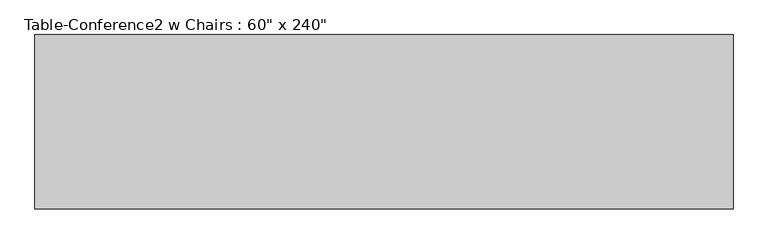
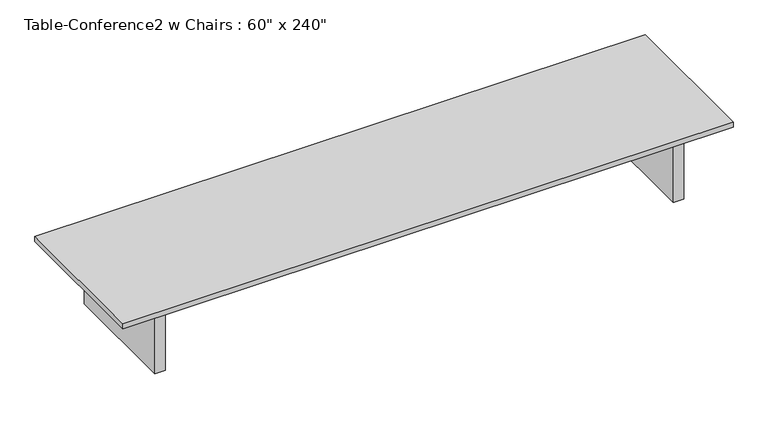
"""IFC4 building model written with IfcOpenShell, lengths in millimetres: furniture geometry."""

import ifcopenshell
import ifcopenshell.guid

model = None  # the IFC model being written
_history = None  # IfcOwnerHistory: only IFC2X3 demands one
_inside = {}  # id of a spatial element -> (the spatial element, [elements in it])
_under = {}  # id of a project, library or spatial element -> (it, [spatial elements below it])
_declared = {}  # id of a project -> (the project, [libraries it declares])
_typed = {}  # id of a type object -> (the type object, [elements of that type])
_made_of = {}  # id of a material, layer set ... -> (it, [elements and type objects made of it])


def new_model(schema):
    """Start an empty IFC model of exactly this schema.

    Asked for "IFC4X3", IfcOpenShell would pick the latest addendum, in which some entities
    have other attributes; the version numbers below select the first issue.
    IFC2X3 requires an IfcOwnerHistory on every rooted entity: one is made here for all.
    """
    global model, _history
    if schema == "IFC4X3":
        model = ifcopenshell.file(schema_version=(4, 3, 0, 0))
    else:
        model = ifcopenshell.file(schema=schema)
    _inside.clear()
    _under.clear()
    _declared.clear()
    _typed.clear()
    _made_of.clear()
    _history = None
    if model.schema == "IFC2X3":
        org = make("IfcOrganization", Name="unknown")
        user = make(
            "IfcPersonAndOrganization",
            ThePerson=make("IfcPerson", FamilyName="unknown"),
            TheOrganization=org,
        )
        app = make(
            "IfcApplication",
            ApplicationDeveloper=org,
            Version="unknown",
            ApplicationFullName="unknown",
            ApplicationIdentifier="unknown",
        )
        _history = make(
            "IfcOwnerHistory",
            OwningUser=user,
            OwningApplication=app,
            ChangeAction="ADDED",
            CreationDate=0,
        )
    return model


def make(cls, **values):
    """One entity of the class cls with the attributes given. An attribute that is None is left unset."""
    return model.create_entity(
        cls, **{name: value for name, value in values.items() if value is not None}
    )


def rooted(cls, **values):
    """An entity with a GlobalId (a new one), such as an element, a storey or a relation."""
    return make(cls, GlobalId=ifcopenshell.guid.new(), OwnerHistory=_history, **values)


def si_unit(unit_type, name, prefix=None):
    """IfcSIUnit, for example si_unit("LENGTHUNIT", "METRE", prefix="MILLI")."""
    return make("IfcSIUnit", UnitType=unit_type, Prefix=prefix, Name=name)


def assignment(units):
    """IfcUnitAssignment: the units of a project."""
    return None if units is None else make("IfcUnitAssignment", Units=units)


def point(xyz):
    """IfcCartesianPoint."""
    return None if xyz is None else make("IfcCartesianPoint", Coordinates=xyz)


def direction(xyz):
    """IfcDirection."""
    return None if xyz is None else make("IfcDirection", DirectionRatios=xyz)


def frame(location, z_axis=None, x_axis=None):
    """IfcAxis2Placement3D, a coordinate frame: its origin and axes. An axis left out is left unset."""
    return make(
        "IfcAxis2Placement3D",
        Location=point(location),
        Axis=direction(z_axis),
        RefDirection=direction(x_axis),
    )


def origin():
    """The frame at (0, 0, 0) with its axes left unset."""
    return frame((0.0, 0.0, 0.0))


def origin_with_axes():
    """The frame at (0, 0, 0) with the z axis (0, 0, 1) and the x axis (1, 0, 0) written out."""
    return frame((0.0, 0.0, 0.0), z_axis=(0.0, 0.0, 1.0), x_axis=(1.0, 0.0, 0.0))


def place(relative_to, where):
    """IfcLocalPlacement: puts the frame where relative to a parent placement (None: the world)."""
    return make(
        "IfcLocalPlacement", PlacementRelTo=relative_to, RelativePlacement=where
    )


def context(
    kind, dimensions, precision=None, world=None, true_north=None, identifier=None
):
    """IfcGeometricRepresentationContext, for example the 3D "Model" context."""
    return make(
        "IfcGeometricRepresentationContext",
        ContextIdentifier=identifier,
        ContextType=kind,
        CoordinateSpaceDimension=dimensions,
        Precision=precision,
        WorldCoordinateSystem=world,
        TrueNorth=true_north,
    )


def project(units=None, contexts=None):
    """IfcProject with its units and contexts."""
    return rooted(
        "IfcProject",
        Name="project",
        RepresentationContexts=contexts,
        UnitsInContext=assignment(units),
    )


def spatial(cls, under=None, at=None, **own):
    """A site, building, storey or space (cls), placed at a placement, below another one or the project."""
    s = rooted(cls, ObjectPlacement=at, **own)
    if under is not None:
        _under.setdefault(under.id(), (under, []))[1].append(s)
    return s


def polyline(points):
    """IfcPolyline through the points."""
    return make("IfcPolyline", Points=[point(p) for p in points])


def outline(outer, holes=None, kind="AREA"):
    """IfcArbitraryClosedProfileDef: a profile drawn as a closed curve; with holes, ...WithVoids."""
    if holes is None:
        return make("IfcArbitraryClosedProfileDef", ProfileType=kind, OuterCurve=outer)
    return make(
        "IfcArbitraryProfileDefWithVoids",
        ProfileType=kind,
        OuterCurve=outer,
        InnerCurves=holes,
    )


def extrude(swept, where, along, depth):
    """IfcExtrudedAreaSolid: the profile swept, set in the frame where, extruded along a direction by depth."""
    return make(
        "IfcExtrudedAreaSolid",
        SweptArea=swept,
        Position=where,
        ExtrudedDirection=direction(along),
        Depth=depth,
    )


def shape(context_of_items, identifier, shape_type, items):
    """IfcShapeRepresentation: the items that make up one representation, for example the "Body"."""
    return make(
        "IfcShapeRepresentation",
        ContextOfItems=context_of_items,
        RepresentationIdentifier=identifier,
        RepresentationType=shape_type,
        Items=items,
    )


def source(mapping_origin, context_of_items, identifier, shape_type, items):
    """IfcRepresentationMap: a shape defined once, which mapped items show again and again."""
    return make(
        "IfcRepresentationMap",
        MappingOrigin=mapping_origin,
        MappedRepresentation=shape(context_of_items, identifier, shape_type, items),
    )


def transform(
    local_origin,
    x_axis=None,
    y_axis=None,
    z_axis=None,
    scale=None,
    scale2=None,
    scale3=None,
    uniform=True,
):
    """IfcCartesianTransformationOperator3D, or its non-uniform kind. x_axis, y_axis, z_axis: its Axis1, 2, 3."""
    if uniform:
        return make(
            "IfcCartesianTransformationOperator3D",
            Axis1=direction(x_axis),
            Axis2=direction(y_axis),
            LocalOrigin=point(local_origin),
            Scale=scale,
            Axis3=direction(z_axis),
        )
    return make(
        "IfcCartesianTransformationOperator3DnonUniform",
        Axis1=direction(x_axis),
        Axis2=direction(y_axis),
        LocalOrigin=point(local_origin),
        Scale=scale,
        Axis3=direction(z_axis),
        Scale2=scale2,
        Scale3=scale3,
    )


def mapped(mapping_source, mapping_target):
    """IfcMappedItem: shows the shape of a source again, moved by a transform."""
    return make(
        "IfcMappedItem", MappingSource=mapping_source, MappingTarget=mapping_target
    )


def made_of(thing, what):
    """Note that an element or type object is made of a material, layer set ...; save() writes the relation."""
    if what is not None:
        _made_of.setdefault(what.id(), (what, []))[1].append(thing)
    return thing


def element(
    cls,
    number,
    at=None,
    inside=None,
    cuts=None,
    type_object=None,
    material=None,
    context=None,
    identifier="Body",
    shape_type=None,
    held_by="IfcProductDefinitionShape",
    body=None,
    shapes=None,
    **own,
):
    """One element of the class cls, such as IfcWall. Its Tag is "e" and its number.

    at: its placement. inside: the storey or other place that contains it. cuts: it is an
    opening in that element (IfcRelVoidsElement). A single representation is given by context,
    identifier, shape_type and body (its items); several are given by shapes. held_by: the class
    of the entity that holds the representations. save() writes the other relations.
    """
    e = rooted(cls, Tag="e%d" % number, ObjectPlacement=at, **own)
    if body is not None:
        shapes = [shape(context, identifier, shape_type, body)]
    if shapes is not None:
        e.Representation = make(held_by, Representations=shapes)
    if inside is not None:
        _inside.setdefault(inside.id(), (inside, []))[1].append(e)
    if cuts is not None:
        rooted(
            "IfcRelVoidsElement", RelatingBuildingElement=cuts, RelatedOpeningElement=e
        )
    if type_object is not None:
        _typed.setdefault(type_object.id(), (type_object, []))[1].append(e)
    return made_of(e, material)


def aggregate(whole, parts):
    """IfcRelAggregates: a whole, such as a stair, and the parts it consists of."""
    return rooted("IfcRelAggregates", RelatingObject=whole, RelatedObjects=parts)


def save(model, path):
    """Write the relations noted so far, then the file.

    IfcRelAggregates (storeys below a building ...), IfcRelContainedInSpatialStructure (elements
    in a storey), IfcRelDefinesByType, IfcRelAssociatesMaterial and IfcRelDeclares: one each for
    every whole, place, type object, material and project.
    """
    for whole, parts in _under.values():
        aggregate(whole, parts)
    for where, things in _inside.values():
        rooted(
            "IfcRelContainedInSpatialStructure",
            RelatedElements=things,
            RelatingStructure=where,
        )
    for kind, things in _typed.values():
        rooted("IfcRelDefinesByType", RelatedObjects=things, RelatingType=kind)
    for what, things in _made_of.values():
        rooted("IfcRelAssociatesMaterial", RelatedObjects=things, RelatingMaterial=what)
    for by, libraries in _declared.values():
        rooted("IfcRelDeclares", RelatingContext=by, RelatedDefinitions=libraries)
    model.write(path)


def furniture_b1813a45(model_context):
    return source(origin(), model_context, "Body", "SweptSolid", [
        extrude(outline(polyline([(2540.0, 609.6), (2540.0, 571.5), (-2540.0, 571.5), (-2540.0, 609.6), (2540.0, 609.6)])), frame((0.0, 0.0, 609.6), z_axis=(0.0, 0.0, 1.0), x_axis=(1.0, 0.0, 0.0)), (0.0, 0.0, 1.0), 101.6),
        extrude(outline(polyline([(2540.0, -609.6), (-2540.0, -609.6), (-2540.0, -571.5), (2540.0, -571.5), (2540.0, -609.6)])), frame((0.0, 0.0, 609.6), z_axis=(0.0, 0.0, 1.0), x_axis=(1.0, 0.0, 0.0)), (0.0, 0.0, 1.0), 101.6),
        extrude(outline(polyline([(-2540.0, -609.6), (-2641.6, -609.6), (-2641.6, 609.6), (-2540.0, 609.6), (-2540.0, -609.6)])), origin_with_axes(), (0.0, 0.0, 1.0), 711.2),
        extrude(outline(polyline([(2641.6, -609.6), (2540.0, -609.6), (2540.0, 609.6), (2641.6, 609.6), (2641.6, -609.6)])), origin_with_axes(), (0.0, 0.0, 1.0), 711.2),
        extrude(outline(polyline([(3048.0, -762.0), (-3048.0, -762.0), (-3048.0, 762.0), (3048.0, 762.0), (3048.0, -762.0)])), frame((0.0, 0.0, 711.2), z_axis=(0.0, 0.0, 1.0), x_axis=(1.0, 0.0, 0.0)), (0.0, 0.0, 1.0), 50.8),
    ])


if __name__ == "__main__":
    model = new_model("IFC4")
    model_context = context("Model", 3, world=origin())
    ifc_project = project(units=[si_unit("LENGTHUNIT", "METRE", prefix="MILLI")], contexts=[model_context])
    site = spatial("IfcSite", under=ifc_project)
    building = spatial("IfcBuilding", under=site)
    placement = place(None, origin())
    furniture_shape = furniture_b1813a45(model_context)
    element("IfcFurniture", 1, ObjectType="Table-Conference2 w Chairs : 60\" x 240\"", at=placement, inside=building, context=model_context, shape_type="MappedRepresentation", body=[
        mapped(furniture_shape, transform((0.0, 0.0, 0.0), x_axis=(1.0, 0.0, 0.0), y_axis=(0.0, 1.0, 0.0), z_axis=(0.0, 0.0, 1.0))),
    ])
    save(model, "model.ifc")

# Revit data of these elements
# Type "Table-Conference2 w Chairs : 60\" x 240\""
#   Type IfcGUID = "2u0XNFrAPALBFZCv81fqiU"
#   Assembly Code = "E2020200"
#   Description = "Seating 20-22"
#   Height = 0.762 m
#   Length = 6.096 m
#   Width = 1.524 m
#   Number Of Chairs One Side = 9
#   Number Of Chairs = 20
#   Material = Wood - Cherry
#   Default Elevation = 0
# Element 1 (IfcFurniture, "Table-Conference2 w Chairs : 60\" x 240\"")
#   Materials on its faces: "Wood - Cherry"
# Materials
#   "Wood - Cherry": class "Wood", colour RGB 226 177 128, transparency 0
